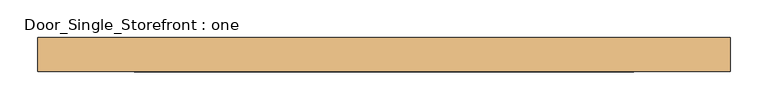
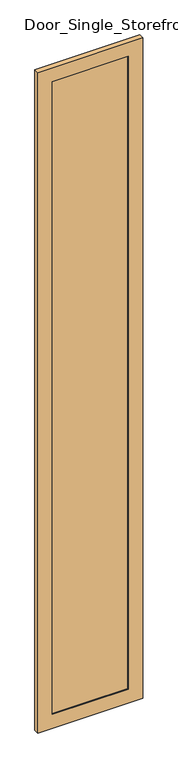
"""IFC4 building model written with IfcOpenShell, lengths in millimetres: door geometry, Door_Single_Storefront : one."""

from ifc_helpers import new_model, si_unit, frame, origin, place, context, project, spatial, polyline, outline, extrude, source, transform, mapped, element, save


def door_single_storefront_one_78bfd28b(model_context):
    return source(origin(), model_context, "Body", "SweptSolid", [
        extrude(outline(polyline([(330.2, -6.35), (-330.2, -6.35), (-330.2, 12.7), (330.2, 12.7), (330.2, -6.35)])), frame((0.0, 0.0, 127.0), z_axis=(0.0, 0.0, 1.0), x_axis=(1.0, 0.0, 0.0)), (0.0, 0.0, 1.0), 5835.65),
        extrude(outline(polyline([(6089.65, -457.2), (0.0, -457.2), (0.0, 457.2), (6089.65, 457.2), (6089.65, -457.2)]), holes=[polyline([(127.0, 330.2), (127.0, -330.2), (5962.65, -330.2), (5962.65, 330.2), (127.0, 330.2)])]), frame((0.0, -19.05, 0.0), z_axis=(0.0, 1.0, 0.0), x_axis=(0.0, 0.0, 1.0)), (0.0, 0.0, 1.0), 44.45),
    ])


if __name__ == "__main__":
    model = new_model("IFC4")
    model_context = context("Model", 3, world=origin())
    ifc_project = project(units=[si_unit("LENGTHUNIT", "METRE", prefix="MILLI")], contexts=[model_context])
    site = spatial("IfcSite", under=ifc_project)
    building = spatial("IfcBuilding", under=site)
    placement = place(None, origin())
    door_single_storefront_one_shape = door_single_storefront_one_78bfd28b(model_context)
    element("IfcDoor", 1, ObjectType="Door_Single_Storefront : one", at=placement, inside=building, context=model_context, shape_type="MappedRepresentation", body=[
        mapped(door_single_storefront_one_shape, transform((0.0, 0.0, 0.0), x_axis=(1.0, 0.0, 0.0), y_axis=(0.0, 1.0, 0.0), z_axis=(0.0, 0.0, 1.0))),
    ])
    save(model, "model.ifc")

# Revit data of these elements
# Type "Door_Single_Storefront : one"
#   Type Mark = "107"
#   Analytic Construction = "<None>"
#   Stile_Width = 0' - 5"
#   Door_Thickness = 0' - 1 3/4"
#   Door_Offset = 0' - 1"
#   Glass_Material = TEMPERED, INSULATED GLASS
#   Frame_Material = EXISTING STOREFRONT
#   Function = (empty or 0)
# Element 1 (IfcDoor, "Door_Single_Storefront : one")
#   Materials on its faces: "EXISTING STOREFRONT", "TEMPERED, INSULATED GLASS"
# Materials
#   "TEMPERED, INSULATED GLASS": class "Glass", colour RGB 214 219 226, transparency 0, Description = "Soda Lime Glass", Cost = 0
#   "EXISTING STOREFRONT": class "Metal", colour RGB 244 244 244, transparency 0, Description = "Aluminum 6061", Cost = 0
